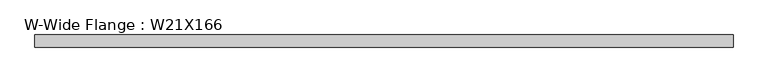
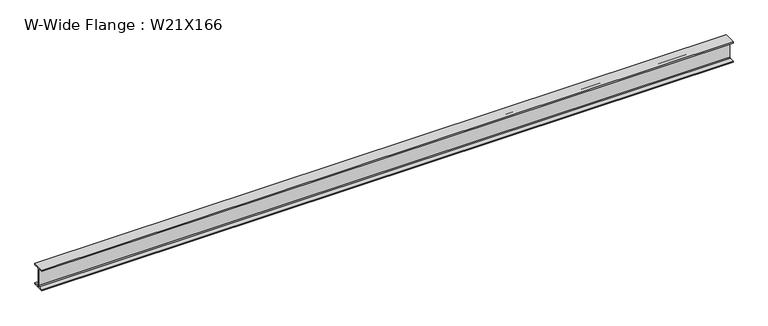
"""IFC4 building model written with IfcOpenShell, lengths in millimetres: beam geometry, W-Wide Flange : W21X166."""

from ifc_helpers import new_model, si_unit, point, frame, frame_2d, origin, place, context, project, spatial, polyline, circle_curve, trimmed, segment, composite_curve, outline, extrude, source, transform, mapped, element, save


def w_wide_flange_w21x166_3b29eaba(model_context):
    return source(origin(), model_context, "Body", "SweptSolid", [
        extrude(outline(composite_curve([segment(polyline([(157.48, -251.206), (157.48, -285.75), (-157.48, -285.75), (-157.48, -251.206), (-32.131, -251.206)]), True, "CONTINUOUS"), segment(trimmed(circle_curve(frame_2d((-32.131, -228.6)), 22.606), [point((-32.131, -251.206))], [point((-9.525, -228.6))], True, "CARTESIAN"), True, "CONTINUOUS"), segment(polyline([(-9.525, -228.6), (-9.525, 228.6)]), True, "CONTINUOUS"), segment(trimmed(circle_curve(frame_2d((-32.131, 228.6)), 22.606), [point((-9.525, 228.6))], [point((-32.131, 251.206))], True, "CARTESIAN"), True, "CONTINUOUS"), segment(polyline([(-32.131, 251.206), (-157.48, 251.206), (-157.48, 285.75), (157.48, 285.75), (157.48, 251.206), (32.131, 251.206)]), True, "CONTINUOUS"), segment(trimmed(circle_curve(frame_2d((32.131, 228.6)), 22.606), [point((32.131, 251.206))], [point((9.525, 228.6))], True, "CARTESIAN"), True, "CONTINUOUS"), segment(polyline([(9.525, 228.6), (9.525, -228.6)]), True, "CONTINUOUS"), segment(trimmed(circle_curve(frame_2d((32.131, -228.6)), 22.606), [point((9.525, -228.6))], [point((32.131, -251.206))], True, "CARTESIAN"), True, "CONTINUOUS"), segment(polyline([(32.131, -251.206), (157.48, -251.206)]), True, "CONTINUOUS")], self_intersect=False)), frame((-9110.634264, 0.0, 0.0), z_axis=(1.0, 0.0, 0.0), x_axis=(0.0, 1.0, 0.0)), (0.0, 0.0, 1.0), 18150.0379668),
    ])


if __name__ == "__main__":
    model = new_model("IFC4")
    model_context = context("Model", 3, world=origin())
    ifc_project = project(units=[si_unit("LENGTHUNIT", "METRE", prefix="MILLI")], contexts=[model_context])
    site = spatial("IfcSite", under=ifc_project)
    building = spatial("IfcBuilding", under=site)
    placement = place(None, origin())
    w_wide_flange_w21x166_shape = w_wide_flange_w21x166_3b29eaba(model_context)
    element("IfcBeam", 1, ObjectType="W-Wide Flange : W21X166", at=placement, inside=building, context=model_context, shape_type="MappedRepresentation", body=[
        mapped(w_wide_flange_w21x166_shape, transform((0.0, 0.0, 0.0), x_axis=(1.0, 0.0, 0.0), y_axis=(0.0, 1.0, 0.0), z_axis=(0.0, 0.0, 1.0))),
    ])
    save(model, "model.ifc")

# Revit data of these elements
# Type "W-Wide Flange : W21X166"
#   Assembly Code = "B10"
#   W = 166
#   Length [instance default] = 5' - 0"
#   bf = 1' - 0.4"
#   d = 1' - 10 1/2"
#   k = 0' - 2 1/4"
#   k2 = 0' - 0.89"
#   tf = 0' - 1.36"
#   tw = 0' - 0 3/4"
#   A = 0.338889 SF
#   Structural Material [instance default] = Steel ASTM A992
# Element 1 (IfcBeam, "W-Wide Flange : W21X166")
#   Structural Material = Steel
#   Materials on its faces: "Steel"
# Materials
#   "Steel ASTM A992": class "Metal", colour RGB 199 199 199, transparency 0, Description = "Structural steel 50ksi", Cost = 0
#   "Steel": class "Metal", colour RGB 118 118 114, transparency 0, Description = "Steel, mill finish", Cost = 0
